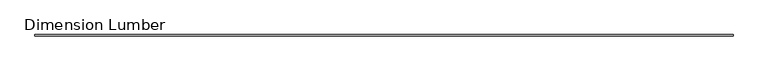
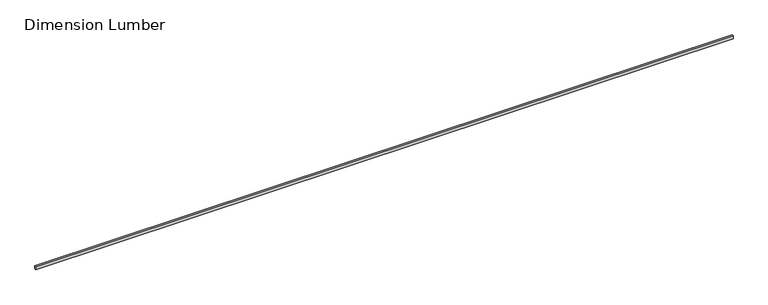
"""IFC4 building model written with IfcOpenShell, lengths in millimetres: beam geometry, Dimension Lumber : Roof Lumbers."""

from ifc_helpers import new_model, si_unit, frame, origin, place, context, project, spatial, polyline, outline, extrude, source, transform, mapped, element, save


def dimension_lumber_f19b9f83(model_context):
    return source(origin(), model_context, "Body", "SweptSolid", [
        extrude(outline(polyline([(13763.625, -19.05), (-5743.575, -19.05), (-5743.575, 19.05), (13763.625, 19.05), (13763.625, -19.05)])), frame((0.0, 0.0, -44.45), z_axis=(0.0, 0.0, 1.0), x_axis=(1.0, 0.0, 0.0)), (0.0, 0.0, 1.0), 88.9),
    ])


if __name__ == "__main__":
    model = new_model("IFC4")
    model_context = context("Model", 3, world=origin())
    ifc_project = project(units=[si_unit("LENGTHUNIT", "METRE", prefix="MILLI")], contexts=[model_context])
    site = spatial("IfcSite", under=ifc_project)
    building = spatial("IfcBuilding", under=site)
    placement = place(None, origin())
    dimension_lumber_shape = dimension_lumber_f19b9f83(model_context)
    element("IfcBeam", 1, ObjectType="Dimension Lumber : Roof Lumbers", at=placement, inside=building, context=model_context, shape_type="MappedRepresentation", body=[
        mapped(dimension_lumber_shape, transform((0.0, 0.0, 0.0), x_axis=(1.0, 0.0, 0.0), y_axis=(0.0, 1.0, 0.0), z_axis=(0.0, 0.0, 1.0))),
    ])
    save(model, "model.ifc")

# Revit data of these elements
# Type "Dimension Lumber : Roof Lumbers"
#   Assembly Code = "B10"
#   A = 0.0364583 SF
#   Length [instance default] = 5' - 0"
#   b = 0' - 1 1/2"
#   d = 0' - 3 1/2"
#   Structural Material [instance default] = Softwood, Lumber
# Element 1 (IfcBeam, "Dimension Lumber : Roof Lumbers")
#   Structural Material = Douglas Fir #2
#   Materials on its faces: "Douglas Fir #2"
# Materials
#   "Softwood, Lumber": class "Wood", colour RGB 223 192 134, transparency 0, Description = "Pinus Echinata", Cost = 0
#   "Douglas Fir #2": class "Wood", colour RGB 223 192 134, transparency 0, Description = "Pinus Echinata", Cost = 0
